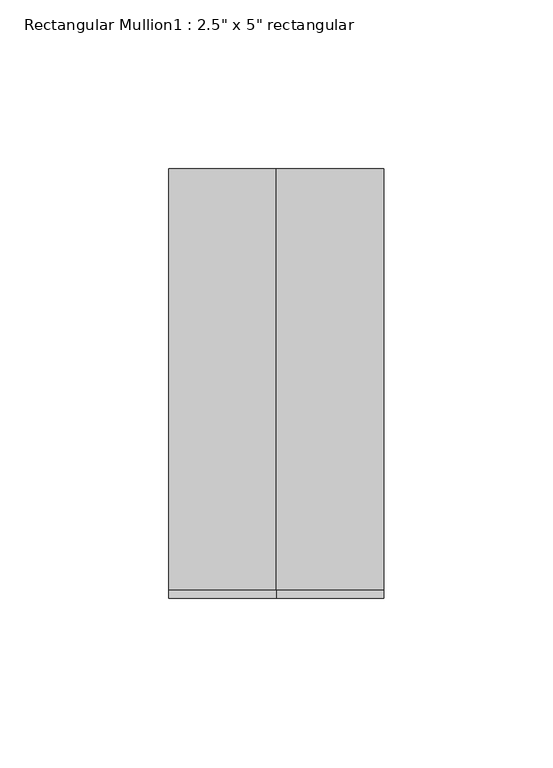
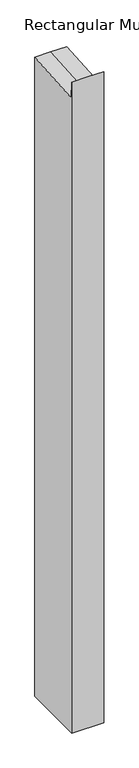
"""IFC4 building model written with IfcOpenShell, lengths in millimetres: member geometry."""

import ifcopenshell
import ifcopenshell.guid

model = None  # the IFC model being written
_history = None  # IfcOwnerHistory: only IFC2X3 demands one
_inside = {}  # id of a spatial element -> (the spatial element, [elements in it])
_under = {}  # id of a project, library or spatial element -> (it, [spatial elements below it])
_declared = {}  # id of a project -> (the project, [libraries it declares])
_typed = {}  # id of a type object -> (the type object, [elements of that type])
_made_of = {}  # id of a material, layer set ... -> (it, [elements and type objects made of it])


def new_model(schema):
    """Start an empty IFC model of exactly this schema.

    Asked for "IFC4X3", IfcOpenShell would pick the latest addendum, in which some entities
    have other attributes; the version numbers below select the first issue.
    IFC2X3 requires an IfcOwnerHistory on every rooted entity: one is made here for all.
    """
    global model, _history
    if schema == "IFC4X3":
        model = ifcopenshell.file(schema_version=(4, 3, 0, 0))
    else:
        model = ifcopenshell.file(schema=schema)
    _inside.clear()
    _under.clear()
    _declared.clear()
    _typed.clear()
    _made_of.clear()
    _history = None
    if model.schema == "IFC2X3":
        org = make("IfcOrganization", Name="unknown")
        user = make(
            "IfcPersonAndOrganization",
            ThePerson=make("IfcPerson", FamilyName="unknown"),
            TheOrganization=org,
        )
        app = make(
            "IfcApplication",
            ApplicationDeveloper=org,
            Version="unknown",
            ApplicationFullName="unknown",
            ApplicationIdentifier="unknown",
        )
        _history = make(
            "IfcOwnerHistory",
            OwningUser=user,
            OwningApplication=app,
            ChangeAction="ADDED",
            CreationDate=0,
        )
    return model


def make(cls, **values):
    """One entity of the class cls with the attributes given. An attribute that is None is left unset."""
    return model.create_entity(
        cls, **{name: value for name, value in values.items() if value is not None}
    )


def rooted(cls, **values):
    """An entity with a GlobalId (a new one), such as an element, a storey or a relation."""
    return make(cls, GlobalId=ifcopenshell.guid.new(), OwnerHistory=_history, **values)


def si_unit(unit_type, name, prefix=None):
    """IfcSIUnit, for example si_unit("LENGTHUNIT", "METRE", prefix="MILLI")."""
    return make("IfcSIUnit", UnitType=unit_type, Prefix=prefix, Name=name)


def assignment(units):
    """IfcUnitAssignment: the units of a project."""
    return None if units is None else make("IfcUnitAssignment", Units=units)


def point(xyz):
    """IfcCartesianPoint."""
    return None if xyz is None else make("IfcCartesianPoint", Coordinates=xyz)


def direction(xyz):
    """IfcDirection."""
    return None if xyz is None else make("IfcDirection", DirectionRatios=xyz)


def frame(location, z_axis=None, x_axis=None):
    """IfcAxis2Placement3D, a coordinate frame: its origin and axes. An axis left out is left unset."""
    return make(
        "IfcAxis2Placement3D",
        Location=point(location),
        Axis=direction(z_axis),
        RefDirection=direction(x_axis),
    )


def origin():
    """The frame at (0, 0, 0) with its axes left unset."""
    return frame((0.0, 0.0, 0.0))


def place(relative_to, where):
    """IfcLocalPlacement: puts the frame where relative to a parent placement (None: the world)."""
    return make(
        "IfcLocalPlacement", PlacementRelTo=relative_to, RelativePlacement=where
    )


def context(
    kind, dimensions, precision=None, world=None, true_north=None, identifier=None
):
    """IfcGeometricRepresentationContext, for example the 3D "Model" context."""
    return make(
        "IfcGeometricRepresentationContext",
        ContextIdentifier=identifier,
        ContextType=kind,
        CoordinateSpaceDimension=dimensions,
        Precision=precision,
        WorldCoordinateSystem=world,
        TrueNorth=true_north,
    )


def project(units=None, contexts=None):
    """IfcProject with its units and contexts."""
    return rooted(
        "IfcProject",
        Name="project",
        RepresentationContexts=contexts,
        UnitsInContext=assignment(units),
    )


def spatial(cls, under=None, at=None, **own):
    """A site, building, storey or space (cls), placed at a placement, below another one or the project."""
    s = rooted(cls, ObjectPlacement=at, **own)
    if under is not None:
        _under.setdefault(under.id(), (under, []))[1].append(s)
    return s


def faces_of(points, faces, orient=None, outer=None):
    """IfcFace entities. A face is a list of loops; a loop is a list of indices into points, from 0.

    orient and outer hold one flag for each loop. By default every Orientation is true, the
    first loop of a face is its IfcFaceOuterBound and the others are IfcFaceBound.
    """
    made = []
    for i, loops in enumerate(faces):
        bounds = []
        for j, loop in enumerate(loops):
            is_outer = j == 0 if outer is None else outer[i][j]
            bounds.append(
                make(
                    "IfcFaceOuterBound" if is_outer else "IfcFaceBound",
                    Bound=make("IfcPolyLoop", Polygon=[points[k] for k in loop]),
                    Orientation=True if orient is None else orient[i][j],
                )
            )
        made.append(make("IfcFace", Bounds=bounds))
    return made


def faceted_brep(points, faces, orient=None, outer=None, voids=None):
    """IfcFacetedBrep: a solid bounded by flat faces; with voids (closed shells), ...WithVoids."""
    shared = [point(p) for p in points]
    hull = make("IfcClosedShell", CfsFaces=faces_of(shared, faces, orient, outer))
    if voids is None:
        return make("IfcFacetedBrep", Outer=hull)
    return make(
        "IfcFacetedBrepWithVoids",
        Outer=hull,
        Voids=[
            make(cls, CfsFaces=faces_of(shared, fs, o, b)) for cls, fs, o, b in voids
        ],
    )


def shape(context_of_items, identifier, shape_type, items):
    """IfcShapeRepresentation: the items that make up one representation, for example the "Body"."""
    return make(
        "IfcShapeRepresentation",
        ContextOfItems=context_of_items,
        RepresentationIdentifier=identifier,
        RepresentationType=shape_type,
        Items=items,
    )


def source(mapping_origin, context_of_items, identifier, shape_type, items):
    """IfcRepresentationMap: a shape defined once, which mapped items show again and again."""
    return make(
        "IfcRepresentationMap",
        MappingOrigin=mapping_origin,
        MappedRepresentation=shape(context_of_items, identifier, shape_type, items),
    )


def transform(
    local_origin,
    x_axis=None,
    y_axis=None,
    z_axis=None,
    scale=None,
    scale2=None,
    scale3=None,
    uniform=True,
):
    """IfcCartesianTransformationOperator3D, or its non-uniform kind. x_axis, y_axis, z_axis: its Axis1, 2, 3."""
    if uniform:
        return make(
            "IfcCartesianTransformationOperator3D",
            Axis1=direction(x_axis),
            Axis2=direction(y_axis),
            LocalOrigin=point(local_origin),
            Scale=scale,
            Axis3=direction(z_axis),
        )
    return make(
        "IfcCartesianTransformationOperator3DnonUniform",
        Axis1=direction(x_axis),
        Axis2=direction(y_axis),
        LocalOrigin=point(local_origin),
        Scale=scale,
        Axis3=direction(z_axis),
        Scale2=scale2,
        Scale3=scale3,
    )


def mapped(mapping_source, mapping_target):
    """IfcMappedItem: shows the shape of a source again, moved by a transform."""
    return make(
        "IfcMappedItem", MappingSource=mapping_source, MappingTarget=mapping_target
    )


def made_of(thing, what):
    """Note that an element or type object is made of a material, layer set ...; save() writes the relation."""
    if what is not None:
        _made_of.setdefault(what.id(), (what, []))[1].append(thing)
    return thing


def element(
    cls,
    number,
    at=None,
    inside=None,
    cuts=None,
    type_object=None,
    material=None,
    context=None,
    identifier="Body",
    shape_type=None,
    held_by="IfcProductDefinitionShape",
    body=None,
    shapes=None,
    **own,
):
    """One element of the class cls, such as IfcWall. Its Tag is "e" and its number.

    at: its placement. inside: the storey or other place that contains it. cuts: it is an
    opening in that element (IfcRelVoidsElement). A single representation is given by context,
    identifier, shape_type and body (its items); several are given by shapes. held_by: the class
    of the entity that holds the representations. save() writes the other relations.
    """
    e = rooted(cls, Tag="e%d" % number, ObjectPlacement=at, **own)
    if body is not None:
        shapes = [shape(context, identifier, shape_type, body)]
    if shapes is not None:
        e.Representation = make(held_by, Representations=shapes)
    if inside is not None:
        _inside.setdefault(inside.id(), (inside, []))[1].append(e)
    if cuts is not None:
        rooted(
            "IfcRelVoidsElement", RelatingBuildingElement=cuts, RelatedOpeningElement=e
        )
    if type_object is not None:
        _typed.setdefault(type_object.id(), (type_object, []))[1].append(e)
    return made_of(e, material)


def aggregate(whole, parts):
    """IfcRelAggregates: a whole, such as a stair, and the parts it consists of."""
    return rooted("IfcRelAggregates", RelatingObject=whole, RelatedObjects=parts)


def save(model, path):
    """Write the relations noted so far, then the file.

    IfcRelAggregates (storeys below a building ...), IfcRelContainedInSpatialStructure (elements
    in a storey), IfcRelDefinesByType, IfcRelAssociatesMaterial and IfcRelDeclares: one each for
    every whole, place, type object, material and project.
    """
    for whole, parts in _under.values():
        aggregate(whole, parts)
    for where, things in _inside.values():
        rooted(
            "IfcRelContainedInSpatialStructure",
            RelatedElements=things,
            RelatingStructure=where,
        )
    for kind, things in _typed.values():
        rooted("IfcRelDefinesByType", RelatedObjects=things, RelatingType=kind)
    for what, things in _made_of.values():
        rooted("IfcRelAssociatesMaterial", RelatedObjects=things, RelatingMaterial=what)
    for by, libraries in _declared.values():
        rooted("IfcRelDeclares", RelatingContext=by, RelatedDefinitions=libraries)
    model.write(path)


def member_23db0025(model_context):
    return source(origin(), model_context, "Body", "Brep", [
        faceted_brep([(31.75, 63.5, -1339.4207165), (31.75, -63.5, -1339.4207165), (-31.75, -63.5, -1339.4207165), (-31.75, 63.5, -1339.4207165), (-31.75, 63.5, 4.6293267), (0.0, 63.5, 4.6293267), (31.75, 63.5, 4.6293267), (-31.75, -63.5, 29.3948455), (-31.75, -60.9736199, -4.616608), (31.75, -63.5, 29.3948455), (0.0, -63.5, 29.3948455), (31.75, -60.9736199, -4.616608), (0.0, -60.9736199, -4.616608)], [[[0, 1, 2, 3]], [[4, 5, 6, 0, 3]], [[7, 8, 4, 3, 2]], [[9, 10, 7, 2, 1]], [[6, 11, 9, 1, 0]], [[6, 5, 12, 11]], [[5, 4, 8, 12]], [[8, 7, 10, 12]], [[10, 9, 11, 12]]]),
    ])


if __name__ == "__main__":
    model = new_model("IFC4")
    model_context = context("Model", 3, world=origin())
    ifc_project = project(units=[si_unit("LENGTHUNIT", "METRE", prefix="MILLI")], contexts=[model_context])
    site = spatial("IfcSite", under=ifc_project)
    building = spatial("IfcBuilding", under=site)
    placement = place(None, origin())
    member_shape = member_23db0025(model_context)
    element("IfcMember", 1, ObjectType="Rectangular Mullion1 : 2.5\" x 5\" rectangular", at=placement, inside=building, context=model_context, shape_type="MappedRepresentation", body=[
        mapped(member_shape, transform((0.0, 0.0, 0.0), x_axis=(1.0, 0.0, 0.0), y_axis=(0.0, 1.0, 0.0), z_axis=(0.0, 0.0, 1.0))),
    ])
    save(model, "model.ifc")

# Revit data of these elements
# Type "Rectangular Mullion1 : 2.5\" x 5\" rectangular"
#   built-in parameter 1007304 = 0.416667 (stored number, unit not read)
#   built-in parameter 1007301 = 0.104167 (stored number, unit not read)
#   built-in parameter 1007300 = 0.104167 (stored number, unit not read)
# Element 1 (IfcMember, "Rectangular Mullion1 : 2.5\" x 5\" rectangular")
#   Materials on its faces: "support-frame"
# Materials
#   "support-frame": class "Unassigned", colour RGB 233 233 233, transparency 0, Cost = 0
